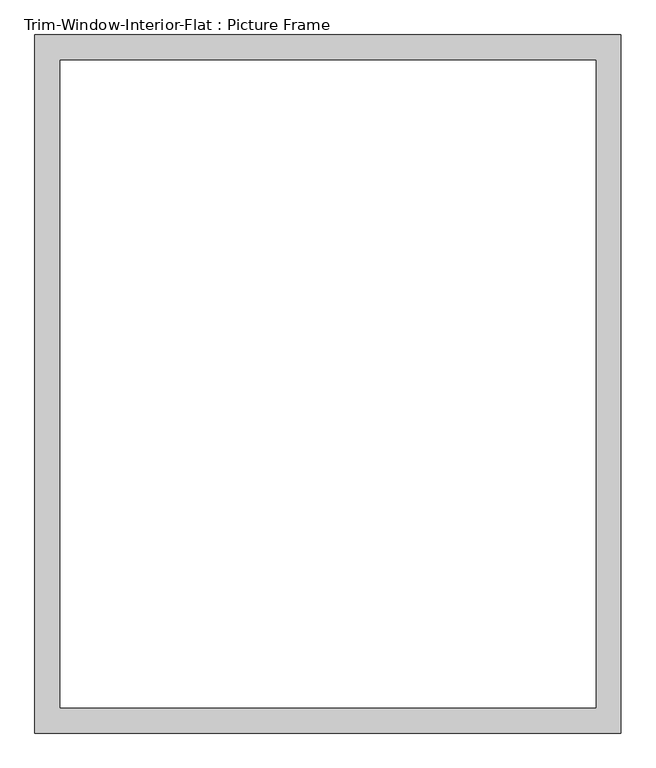
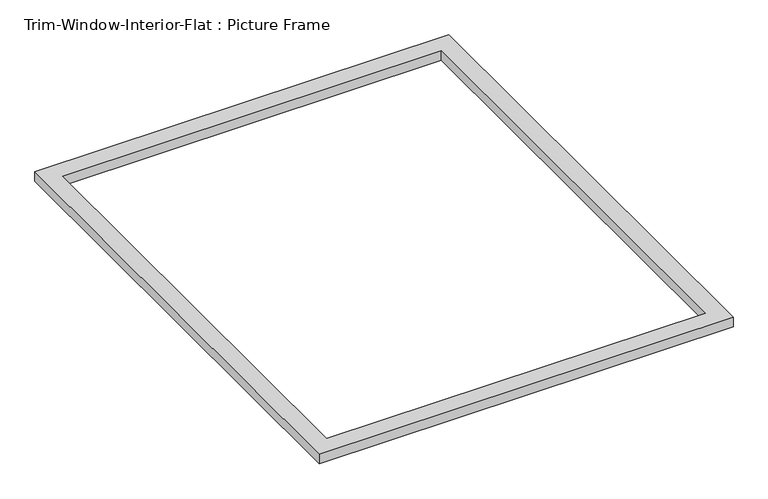
"""IFC4 building model written with IfcOpenShell, lengths in millimetres: proxy geometry, Trim-Window-Interior-Flat : Picture Frame."""

from ifc_helpers import new_model, si_unit, origin, origin_with_axes, place, context, project, spatial, polyline, outline, extrude, source, transform, mapped, element, save


def trim_window_interior_flat_picture_frame_691deff5(model_context):
    return source(origin(), model_context, "Body", "SweptSolid", [
        extrude(outline(polyline([(666.75, 44.45), (666.75, -1543.05), (-666.75, -1543.05), (-666.75, 44.45), (666.75, 44.45)]), holes=[polyline([(609.6, -12.7), (-609.6, -12.7), (-609.6, -1485.9), (609.6, -1485.9), (609.6, -12.7)])]), origin_with_axes(), (0.0, 0.0, 1.0), 31.75),
    ])


if __name__ == "__main__":
    model = new_model("IFC4")
    model_context = context("Model", 3, world=origin())
    ifc_project = project(units=[si_unit("LENGTHUNIT", "METRE", prefix="MILLI")], contexts=[model_context])
    site = spatial("IfcSite", under=ifc_project)
    building = spatial("IfcBuilding", under=site)
    placement = place(None, origin())
    trim_window_interior_flat_picture_frame_shape = trim_window_interior_flat_picture_frame_691deff5(model_context)
    element("IfcBuildingElementProxy", 1, Name="Trim-Window-Interior-Flat : Picture Frame", ObjectType="Trim-Window-Interior-Flat : Picture Frame", at=placement, inside=building, context=model_context, shape_type="MappedRepresentation", body=[
        mapped(trim_window_interior_flat_picture_frame_shape, transform((0.0, 0.0, 0.0), x_axis=(1.0, 0.0, 0.0), y_axis=(0.0, 1.0, 0.0), z_axis=(0.0, 0.0, 1.0))),
    ])
    save(model, "model.ifc")

# Revit data of these elements
# Type "Trim-Window-Interior-Flat : Picture Frame"
#   Trim Thickness_Picture Frame = 0' - 1 1/4"
#   Trim Width = 0' - 2 1/4"
#   Trim Thickness_with Sill = 0' - 0 3/4"
#   Sill Thickness = 0' - 1 1/4"
#   Opening Width [instance default] = 2' - 0"
#   Opening Height [instance default] = 3' - 0"
#   Default Elevation = 4' - 0"
#   Sill = no
#   Picture Frame = yes
#   Trim Material [instance default] = none
# Element 1 (IfcBuildingElementProxy, "Trim-Window-Interior-Flat : Picture Frame")
#   Opening Width = 4' - 1"
#   Opening Height = 4' - 11"
#   Trim Material = 1X WOOD COMPOSITE TRIM
#   Materials on its faces: "1X WOOD COMPOSITE TRIM"
# Materials
#   "1X WOOD COMPOSITE TRIM": class "Generic", colour RGB 88 61 61, transparency 0, Cost = 0
